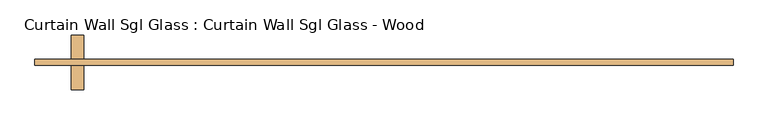
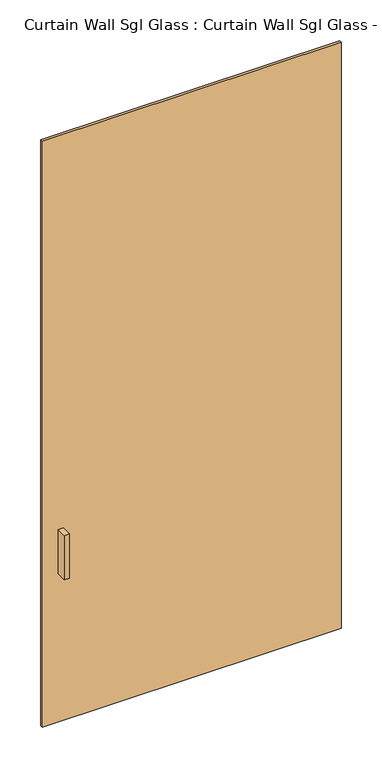
"""IFC4 building model written with IfcOpenShell, lengths in millimetres: door geometry, Curtain Wall Sgl Glass : Curtain Wall Sgl Glass - Wood."""

import ifcopenshell
import ifcopenshell.guid

model = None  # the IFC model being written
_history = None  # IfcOwnerHistory: only IFC2X3 demands one
_inside = {}  # id of a spatial element -> (the spatial element, [elements in it])
_under = {}  # id of a project, library or spatial element -> (it, [spatial elements below it])
_declared = {}  # id of a project -> (the project, [libraries it declares])
_typed = {}  # id of a type object -> (the type object, [elements of that type])
_made_of = {}  # id of a material, layer set ... -> (it, [elements and type objects made of it])


def new_model(schema):
    """Start an empty IFC model of exactly this schema.

    Asked for "IFC4X3", IfcOpenShell would pick the latest addendum, in which some entities
    have other attributes; the version numbers below select the first issue.
    IFC2X3 requires an IfcOwnerHistory on every rooted entity: one is made here for all.
    """
    global model, _history
    if schema == "IFC4X3":
        model = ifcopenshell.file(schema_version=(4, 3, 0, 0))
    else:
        model = ifcopenshell.file(schema=schema)
    _inside.clear()
    _under.clear()
    _declared.clear()
    _typed.clear()
    _made_of.clear()
    _history = None
    if model.schema == "IFC2X3":
        org = make("IfcOrganization", Name="unknown")
        user = make(
            "IfcPersonAndOrganization",
            ThePerson=make("IfcPerson", FamilyName="unknown"),
            TheOrganization=org,
        )
        app = make(
            "IfcApplication",
            ApplicationDeveloper=org,
            Version="unknown",
            ApplicationFullName="unknown",
            ApplicationIdentifier="unknown",
        )
        _history = make(
            "IfcOwnerHistory",
            OwningUser=user,
            OwningApplication=app,
            ChangeAction="ADDED",
            CreationDate=0,
        )
    return model


def make(cls, **values):
    """One entity of the class cls with the attributes given. An attribute that is None is left unset."""
    return model.create_entity(
        cls, **{name: value for name, value in values.items() if value is not None}
    )


def rooted(cls, **values):
    """An entity with a GlobalId (a new one), such as an element, a storey or a relation."""
    return make(cls, GlobalId=ifcopenshell.guid.new(), OwnerHistory=_history, **values)


def si_unit(unit_type, name, prefix=None):
    """IfcSIUnit, for example si_unit("LENGTHUNIT", "METRE", prefix="MILLI")."""
    return make("IfcSIUnit", UnitType=unit_type, Prefix=prefix, Name=name)


def assignment(units):
    """IfcUnitAssignment: the units of a project."""
    return None if units is None else make("IfcUnitAssignment", Units=units)


def point(xyz):
    """IfcCartesianPoint."""
    return None if xyz is None else make("IfcCartesianPoint", Coordinates=xyz)


def direction(xyz):
    """IfcDirection."""
    return None if xyz is None else make("IfcDirection", DirectionRatios=xyz)


def frame(location, z_axis=None, x_axis=None):
    """IfcAxis2Placement3D, a coordinate frame: its origin and axes. An axis left out is left unset."""
    return make(
        "IfcAxis2Placement3D",
        Location=point(location),
        Axis=direction(z_axis),
        RefDirection=direction(x_axis),
    )


def origin():
    """The frame at (0, 0, 0) with its axes left unset."""
    return frame((0.0, 0.0, 0.0))


def origin_with_axes():
    """The frame at (0, 0, 0) with the z axis (0, 0, 1) and the x axis (1, 0, 0) written out."""
    return frame((0.0, 0.0, 0.0), z_axis=(0.0, 0.0, 1.0), x_axis=(1.0, 0.0, 0.0))


def place(relative_to, where):
    """IfcLocalPlacement: puts the frame where relative to a parent placement (None: the world)."""
    return make(
        "IfcLocalPlacement", PlacementRelTo=relative_to, RelativePlacement=where
    )


def context(
    kind, dimensions, precision=None, world=None, true_north=None, identifier=None
):
    """IfcGeometricRepresentationContext, for example the 3D "Model" context."""
    return make(
        "IfcGeometricRepresentationContext",
        ContextIdentifier=identifier,
        ContextType=kind,
        CoordinateSpaceDimension=dimensions,
        Precision=precision,
        WorldCoordinateSystem=world,
        TrueNorth=true_north,
    )


def project(units=None, contexts=None):
    """IfcProject with its units and contexts."""
    return rooted(
        "IfcProject",
        Name="project",
        RepresentationContexts=contexts,
        UnitsInContext=assignment(units),
    )


def spatial(cls, under=None, at=None, **own):
    """A site, building, storey or space (cls), placed at a placement, below another one or the project."""
    s = rooted(cls, ObjectPlacement=at, **own)
    if under is not None:
        _under.setdefault(under.id(), (under, []))[1].append(s)
    return s


def polyline(points):
    """IfcPolyline through the points."""
    return make("IfcPolyline", Points=[point(p) for p in points])


def outline(outer, holes=None, kind="AREA"):
    """IfcArbitraryClosedProfileDef: a profile drawn as a closed curve; with holes, ...WithVoids."""
    if holes is None:
        return make("IfcArbitraryClosedProfileDef", ProfileType=kind, OuterCurve=outer)
    return make(
        "IfcArbitraryProfileDefWithVoids",
        ProfileType=kind,
        OuterCurve=outer,
        InnerCurves=holes,
    )


def extrude(swept, where, along, depth):
    """IfcExtrudedAreaSolid: the profile swept, set in the frame where, extruded along a direction by depth."""
    return make(
        "IfcExtrudedAreaSolid",
        SweptArea=swept,
        Position=where,
        ExtrudedDirection=direction(along),
        Depth=depth,
    )


def shape(context_of_items, identifier, shape_type, items):
    """IfcShapeRepresentation: the items that make up one representation, for example the "Body"."""
    return make(
        "IfcShapeRepresentation",
        ContextOfItems=context_of_items,
        RepresentationIdentifier=identifier,
        RepresentationType=shape_type,
        Items=items,
    )


def source(mapping_origin, context_of_items, identifier, shape_type, items):
    """IfcRepresentationMap: a shape defined once, which mapped items show again and again."""
    return make(
        "IfcRepresentationMap",
        MappingOrigin=mapping_origin,
        MappedRepresentation=shape(context_of_items, identifier, shape_type, items),
    )


def transform(
    local_origin,
    x_axis=None,
    y_axis=None,
    z_axis=None,
    scale=None,
    scale2=None,
    scale3=None,
    uniform=True,
):
    """IfcCartesianTransformationOperator3D, or its non-uniform kind. x_axis, y_axis, z_axis: its Axis1, 2, 3."""
    if uniform:
        return make(
            "IfcCartesianTransformationOperator3D",
            Axis1=direction(x_axis),
            Axis2=direction(y_axis),
            LocalOrigin=point(local_origin),
            Scale=scale,
            Axis3=direction(z_axis),
        )
    return make(
        "IfcCartesianTransformationOperator3DnonUniform",
        Axis1=direction(x_axis),
        Axis2=direction(y_axis),
        LocalOrigin=point(local_origin),
        Scale=scale,
        Axis3=direction(z_axis),
        Scale2=scale2,
        Scale3=scale3,
    )


def mapped(mapping_source, mapping_target):
    """IfcMappedItem: shows the shape of a source again, moved by a transform."""
    return make(
        "IfcMappedItem", MappingSource=mapping_source, MappingTarget=mapping_target
    )


def made_of(thing, what):
    """Note that an element or type object is made of a material, layer set ...; save() writes the relation."""
    if what is not None:
        _made_of.setdefault(what.id(), (what, []))[1].append(thing)
    return thing


def element(
    cls,
    number,
    at=None,
    inside=None,
    cuts=None,
    type_object=None,
    material=None,
    context=None,
    identifier="Body",
    shape_type=None,
    held_by="IfcProductDefinitionShape",
    body=None,
    shapes=None,
    **own,
):
    """One element of the class cls, such as IfcWall. Its Tag is "e" and its number.

    at: its placement. inside: the storey or other place that contains it. cuts: it is an
    opening in that element (IfcRelVoidsElement). A single representation is given by context,
    identifier, shape_type and body (its items); several are given by shapes. held_by: the class
    of the entity that holds the representations. save() writes the other relations.
    """
    e = rooted(cls, Tag="e%d" % number, ObjectPlacement=at, **own)
    if body is not None:
        shapes = [shape(context, identifier, shape_type, body)]
    if shapes is not None:
        e.Representation = make(held_by, Representations=shapes)
    if inside is not None:
        _inside.setdefault(inside.id(), (inside, []))[1].append(e)
    if cuts is not None:
        rooted(
            "IfcRelVoidsElement", RelatingBuildingElement=cuts, RelatedOpeningElement=e
        )
    if type_object is not None:
        _typed.setdefault(type_object.id(), (type_object, []))[1].append(e)
    return made_of(e, material)


def aggregate(whole, parts):
    """IfcRelAggregates: a whole, such as a stair, and the parts it consists of."""
    return rooted("IfcRelAggregates", RelatingObject=whole, RelatedObjects=parts)


def save(model, path):
    """Write the relations noted so far, then the file.

    IfcRelAggregates (storeys below a building ...), IfcRelContainedInSpatialStructure (elements
    in a storey), IfcRelDefinesByType, IfcRelAssociatesMaterial and IfcRelDeclares: one each for
    every whole, place, type object, material and project.
    """
    for whole, parts in _under.values():
        aggregate(whole, parts)
    for where, things in _inside.values():
        rooted(
            "IfcRelContainedInSpatialStructure",
            RelatedElements=things,
            RelatingStructure=where,
        )
    for kind, things in _typed.values():
        rooted("IfcRelDefinesByType", RelatedObjects=things, RelatingType=kind)
    for what, things in _made_of.values():
        rooted("IfcRelAssociatesMaterial", RelatedObjects=things, RelatingMaterial=what)
    for by, libraries in _declared.values():
        rooted("IfcRelDeclares", RelatingContext=by, RelatedDefinitions=libraries)
    model.write(path)


def curtain_wall_sgl_glass_curtain_wall_sgl_glass_wood_e1d2974b(model_context):
    return source(origin(), model_context, "Body", "SweptSolid", [
        extrude(outline(polyline([(-625.475, 12.7), (-625.475, -38.1), (-650.875, -38.1), (-650.875, 12.7), (-625.475, 12.7)])), frame((0.0, 0.0, 762.0), z_axis=(0.0, 0.0, 1.0), x_axis=(1.0, 0.0, 0.0)), (0.0, 0.0, 1.0), 228.6),
        extrude(outline(polyline([(-650.875, -101.6), (-650.875, -50.8), (-625.475, -50.8), (-625.475, -101.6), (-650.875, -101.6)])), frame((0.0, 0.0, 762.0), z_axis=(0.0, 0.0, 1.0), x_axis=(1.0, 0.0, 0.0)), (0.0, 0.0, 1.0), 228.6),
        extrude(outline(polyline([(727.075, -50.8), (-727.075, -50.8), (-727.075, -38.1), (727.075, -38.1), (727.075, -50.8)])), origin_with_axes(), (0.0, 0.0, 1.0), 3016.25),
    ])


if __name__ == "__main__":
    model = new_model("IFC4")
    model_context = context("Model", 3, world=origin())
    ifc_project = project(units=[si_unit("LENGTHUNIT", "METRE", prefix="MILLI")], contexts=[model_context])
    site = spatial("IfcSite", under=ifc_project)
    building = spatial("IfcBuilding", under=site)
    placement = place(None, origin())
    curtain_wall_sgl_glass_curtain_wall_sgl_glass_wood_shape = curtain_wall_sgl_glass_curtain_wall_sgl_glass_wood_e1d2974b(model_context)
    element("IfcDoor", 1, ObjectType="Curtain Wall Sgl Glass : Curtain Wall Sgl Glass - Wood", at=placement, inside=building, context=model_context, shape_type="MappedRepresentation", body=[
        mapped(curtain_wall_sgl_glass_curtain_wall_sgl_glass_wood_shape, transform((0.0, 0.0, 0.0), x_axis=(1.0, 0.0, 0.0), y_axis=(0.0, 1.0, 0.0), z_axis=(0.0, 0.0, 1.0))),
    ])
    save(model, "model.ifc")

# Revit data of these elements
# Project information
#   SR Document GUID = "95f8c40d-21e0-4786-882e-2c1e01a6cca9"
# Type "Curtain Wall Sgl Glass : Curtain Wall Sgl Glass - Wood"
#   Type Mark = "9"
#   Assembly Code = "B2030100"
#   Offset = 0' - 2"
#   Function = 1
#   Handle Material = Metal - Aluminum
#   Glazing Material = Wood Panel - Dark
# Element 1 (IfcDoor, "Curtain Wall Sgl Glass : Curtain Wall Sgl Glass - Wood")
#   Materials on its faces: "Metal - Aluminum", "Wood Panel - Dark"
# Materials
#   "Metal - Aluminum": class "Metal", colour RGB 247 247 247, transparency 0
#   "Wood Panel - Dark": class "Unassigned", colour RGB 57 19 6, transparency 0
